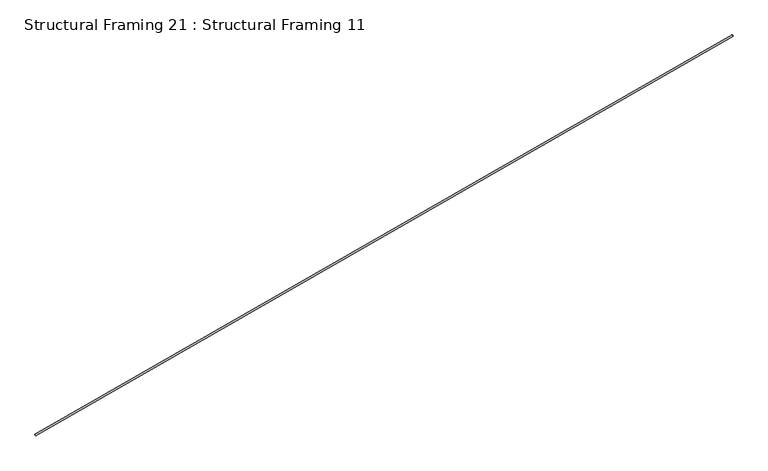
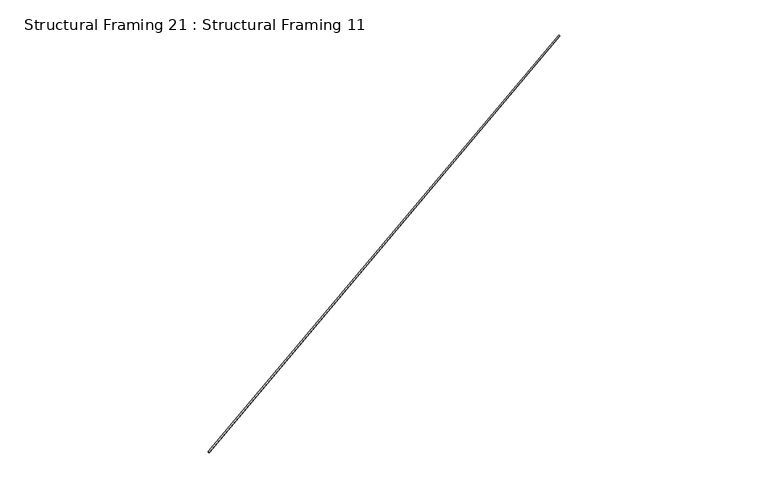
"""IFC4 building model written with IfcOpenShell, lengths in millimetres: beam geometry, Structural Framing 21 : Structural Framing 11."""

from ifc_helpers import new_model, si_unit, point, frame, origin, origin_2d, place, context, project, spatial, circle_curve, trimmed, segment, composite_curve, outline, extrude, source, transform, mapped, element, save


def structural_framing_21_structural_framing_11_394e9749(model_context):
    return source(origin(), model_context, "Body", "SweptSolid", [
        extrude(outline(composite_curve([segment(trimmed(circle_curve(origin_2d(), 6.35), [point((0.0, 6.35))], [point((0.0, -6.35))], False, "CARTESIAN"), True, "CONTINUOUS"), segment(trimmed(circle_curve(origin_2d(), 6.35), [point((0.0, -6.35))], [point((0.0, 6.35))], False, "CARTESIAN"), True, "CONTINUOUS")], self_intersect=False)), frame((23230.1665052, 4180.6567775, 4935.1357581), z_axis=(0.8608596592499228, 0.4936496943962521, 0.12341242359906028), x_axis=(0.0, -0.24253562503632656, 0.9701425001453335)), (0.0, 0.0, 1.0), 5892.4476777),
    ])


if __name__ == "__main__":
    model = new_model("IFC4")
    model_context = context("Model", 3, world=origin())
    ifc_project = project(units=[si_unit("LENGTHUNIT", "METRE", prefix="MILLI")], contexts=[model_context])
    site = spatial("IfcSite", under=ifc_project)
    building = spatial("IfcBuilding", under=site)
    placement = place(None, origin())
    structural_framing_21_structural_framing_11_shape = structural_framing_21_structural_framing_11_394e9749(model_context)
    element("IfcBeam", 1, ObjectType="Structural Framing 21 : Structural Framing 11", at=placement, inside=building, context=model_context, shape_type="MappedRepresentation", body=[
        mapped(structural_framing_21_structural_framing_11_shape, transform((0.0, 0.0, 0.0), x_axis=(1.0, 0.0, 0.0), y_axis=(0.0, 1.0, 0.0), z_axis=(0.0, 0.0, 1.0))),
    ])
    save(model, "model.ifc")

# Revit data of these elements
# Type "Structural Framing 21 : Structural Framing 11"
#   Structural Material [instance default] = EXISTING LATERAL BRACING (1/4" CABLE)
# Element 1 (IfcBeam, "Structural Framing 21 : Structural Framing 11")
#   Materials on its faces: "EXISTING LATERAL BRACING (1/4\" CABLE)"
# Materials
#   "EXISTING LATERAL BRACING (1/4\" CABLE)": class "Generic", colour RGB 120 120 120, transparency 0, Cost = 0
